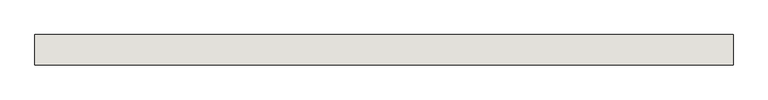
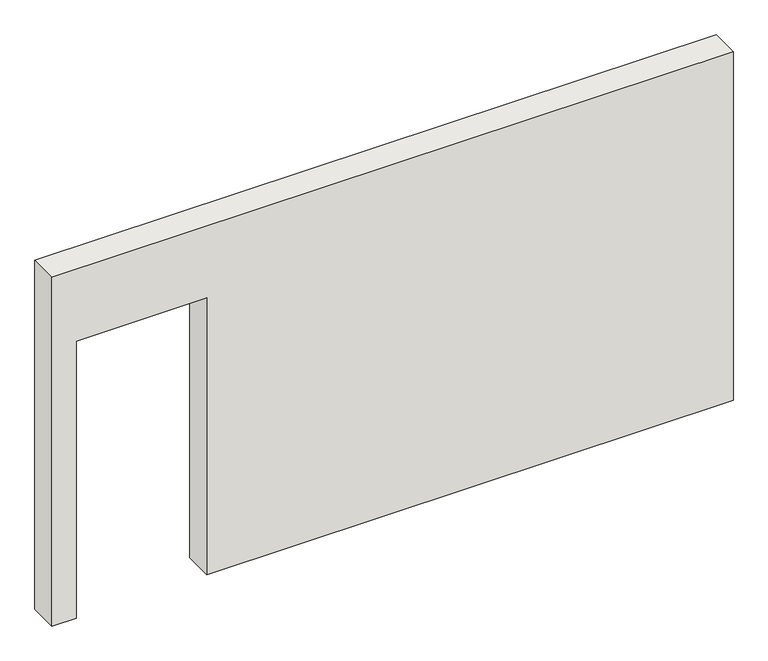
"""IFC4 building model written with IfcOpenShell, lengths in millimetres: wall geometry, Holzwand."""

from ifc_helpers import new_model, si_unit, frame, origin, place, context, project, spatial, polyline, outline, extrude, source, transform, mapped, element, save


def wall_862eeda9(model_context):
    return source(origin(), model_context, "Body", "SweptSolid", [
        extrude(outline(polyline([(1985.0, 1049.2274956), (0.0, 1049.2274956), (0.0, 4620.0), (2500.0, 4620.0), (2500.0, 0.0), (0.0, 0.0), (0.0, 164.2274956), (1985.0, 164.2274956), (1985.0, 1049.2274956)])), frame((0.0, 0.0, 0.0), z_axis=(0.0, 1.0, 0.0), x_axis=(0.0, 0.0, 1.0)), (0.0, 0.0, 1.0), 200.0),
    ])


if __name__ == "__main__":
    model = new_model("IFC4")
    model_context = context("Model", 3, world=origin())
    ifc_project = project(units=[si_unit("LENGTHUNIT", "METRE", prefix="MILLI")], contexts=[model_context])
    site = spatial("IfcSite", under=ifc_project)
    building = spatial("IfcBuilding", under=site)
    placement = place(None, origin())
    wall_shape = wall_862eeda9(model_context)
    element("IfcWall", 1, ObjectType="Holzwand", at=placement, inside=building, context=model_context, shape_type="MappedRepresentation", body=[
        mapped(wall_shape, transform((0.0, 0.0, 0.0), x_axis=(1.0, 0.0, 0.0), y_axis=(0.0, 1.0, 0.0), z_axis=(0.0, 0.0, 1.0))),
    ])
    save(model, "model.ifc")

# Revit data of these elements
# Element 1 (IfcWall, "Holzwand")
#   Materials on its faces: "holzschalung"
# Materials
#   "holzschalung": class "Unassigned", colour RGB 128 128 128, transparency 0
